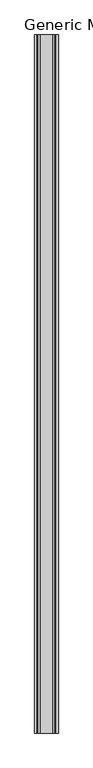
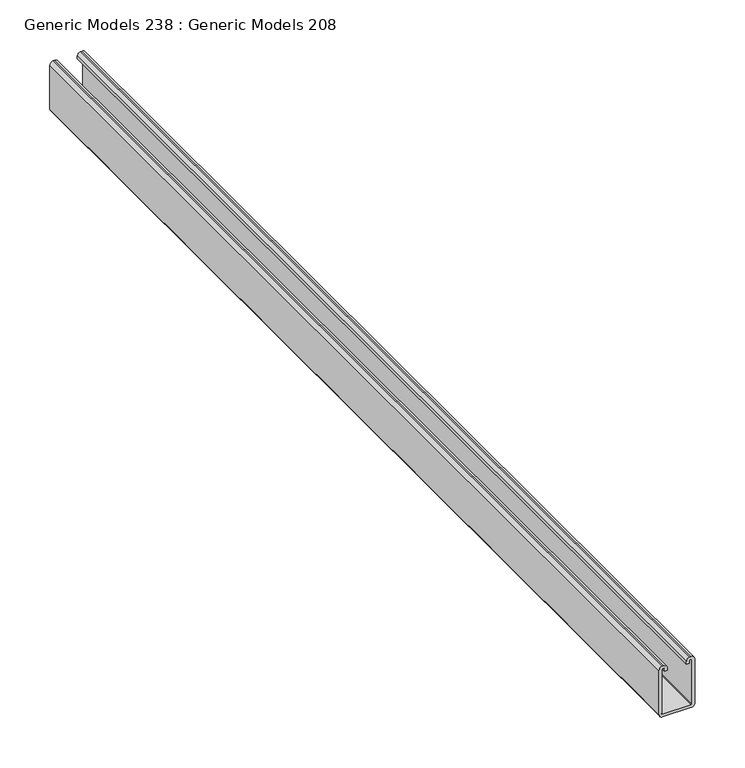
"""IFC4 building model written with IfcOpenShell, lengths in millimetres: proxy geometry, Generic Models 238 : Generic Models 208."""

from ifc_helpers import new_model, si_unit, point, frame, frame_2d, origin, place, context, project, spatial, polyline, circle_curve, trimmed, segment, composite_curve, outline, extrude, source, transform, mapped, element, save


def generic_models_238_generic_models_208_010beb91(model_context):
    return source(origin(), model_context, "Body", "SweptSolid", [
        extrude(outline(composite_curve([segment(polyline([(1885.7283045, 53737.481697), (1882.5378412, 53737.481697), (1882.5378412, 53740.656697), (1885.7283045, 53740.656697)]), True, "CONTINUOUS"), segment(trimmed(circle_curve(frame_2d((1885.7283045, 53741.4349838)), 0.7782868), [point((1885.7283045, 53740.656697))], [point((1886.5065912, 53741.4349838))], True, "CARTESIAN"), True, "CONTINUOUS"), segment(polyline([(1886.5065912, 53741.4349838), (1886.5065912, 53742.9812383)]), True, "CONTINUOUS"), segment(trimmed(circle_curve(frame_2d((1885.6561325, 53742.9812383)), 0.8504588), [point((1886.5065912, 53742.9812383))], [point((1885.6561325, 53743.831697))], True, "CARTESIAN"), True, "CONTINUOUS"), segment(polyline([(1885.6561325, 53743.831697), (1831.7929359, 53743.831697)]), True, "CONTINUOUS"), segment(trimmed(circle_curve(frame_2d((1831.7929359, 53742.9828524)), 0.8488446), [point((1831.7929359, 53743.831697))], [point((1830.9440912, 53742.9828524))], True, "CARTESIAN"), True, "CONTINUOUS"), segment(polyline([(1830.9440912, 53742.9828524), (1830.9440912, 53709.7160199)]), True, "CONTINUOUS"), segment(trimmed(circle_curve(frame_2d((1831.7534142, 53709.7160199)), 0.8093229), [point((1830.9440912, 53709.7160199))], [point((1831.7534142, 53708.906697))], True, "CARTESIAN"), True, "CONTINUOUS"), segment(polyline([(1831.7534142, 53708.906697), (1885.6696823, 53708.906697)]), True, "CONTINUOUS"), segment(trimmed(circle_curve(frame_2d((1885.6696823, 53709.7436059)), 0.8369089), [point((1885.6696823, 53708.906697))], [point((1886.5065912, 53709.7436059))], True, "CARTESIAN"), True, "CONTINUOUS"), segment(polyline([(1886.5065912, 53709.7436059), (1886.5065912, 53711.2123941)]), True, "CONTINUOUS"), segment(trimmed(circle_curve(frame_2d((1885.6372883, 53711.2123941)), 0.8693029), [point((1886.5065912, 53711.2123941))], [point((1885.6372883, 53712.081697))], True, "CARTESIAN"), True, "CONTINUOUS"), segment(polyline([(1885.6372883, 53712.081697), (1882.5378412, 53712.081697), (1882.5378412, 53715.256697), (1885.6372883, 53715.256697)]), True, "CONTINUOUS"), segment(trimmed(circle_curve(frame_2d((1885.6372883, 53711.2123941)), 4.0443029), [point((1885.6372883, 53715.256697))], [point((1889.6815912, 53711.2123941))], False, "CARTESIAN"), True, "CONTINUOUS"), segment(polyline([(1889.6815912, 53711.2123941), (1889.6815912, 53709.7436059)]), True, "CONTINUOUS"), segment(trimmed(circle_curve(frame_2d((1885.6696823, 53709.7436059)), 4.0119089), [point((1889.6815912, 53709.7436059))], [point((1885.6696823, 53705.731697))], False, "CARTESIAN"), True, "CONTINUOUS"), segment(polyline([(1885.6696823, 53705.731697), (1831.7534142, 53705.731697)]), True, "CONTINUOUS"), segment(trimmed(circle_curve(frame_2d((1831.7534142, 53709.7160199)), 3.9843229), [point((1831.7534142, 53705.731697))], [point((1827.7690912, 53709.7160199))], False, "CARTESIAN"), True, "CONTINUOUS"), segment(polyline([(1827.7690912, 53709.7160199), (1827.7690912, 53742.9828524)]), True, "CONTINUOUS"), segment(trimmed(circle_curve(frame_2d((1831.7929359, 53742.9828524)), 4.0238446), [point((1827.7690912, 53742.9828524))], [point((1831.7929359, 53747.006697))], False, "CARTESIAN"), True, "CONTINUOUS"), segment(polyline([(1831.7929359, 53747.006697), (1885.6561325, 53747.006697)]), True, "CONTINUOUS"), segment(trimmed(circle_curve(frame_2d((1885.6561325, 53742.9812383)), 4.0254588), [point((1885.6561325, 53747.006697))], [point((1889.6815912, 53742.9812383))], False, "CARTESIAN"), True, "CONTINUOUS"), segment(polyline([(1889.6815912, 53742.9812383), (1889.6815912, 53741.4349838)]), True, "CONTINUOUS"), segment(trimmed(circle_curve(frame_2d((1885.7283045, 53741.4349838)), 3.9532868), [point((1889.6815912, 53741.4349838))], [point((1885.7283045, 53737.481697))], False, "CARTESIAN"), True, "CONTINUOUS")], self_intersect=False)), frame((0.0, -228.7033818, 0.0), z_axis=(0.0, 1.0, 0.0), x_axis=(0.0, 0.0, 1.0)), (0.0, 0.0, 1.0), 1219.2),
    ])


if __name__ == "__main__":
    model = new_model("IFC4")
    model_context = context("Model", 3, world=origin())
    ifc_project = project(units=[si_unit("LENGTHUNIT", "METRE", prefix="MILLI")], contexts=[model_context])
    site = spatial("IfcSite", under=ifc_project)
    building = spatial("IfcBuilding", under=site)
    placement = place(None, origin())
    generic_models_238_generic_models_208_shape = generic_models_238_generic_models_208_010beb91(model_context)
    element("IfcBuildingElementProxy", 1, Name="Generic Models 238 : Generic Models 208", ObjectType="Generic Models 238 : Generic Models 208", at=placement, inside=building, context=model_context, shape_type="MappedRepresentation", body=[
        mapped(generic_models_238_generic_models_208_shape, transform((0.0, 0.0, 0.0), x_axis=(1.0, 0.0, 0.0), y_axis=(0.0, 1.0, 0.0), z_axis=(0.0, 0.0, 1.0))),
    ])
    save(model, "model.ifc")

# Revit data of these elements
# Element 1 (IfcBuildingElementProxy, "Generic Models 238 : Generic Models 208")
#   Materials on its faces: "GALVANIZED UNISTRUT P5500, 1 5/8\" X 2 7/16\" OR ALUM. CHANNEL"
# Materials
#   "GALVANIZED UNISTRUT P5500, 1 5/8\" X 2 7/16\" OR ALUM. CHANNEL": class "Metal", colour RGB 244 244 244, transparency 0, Description = "Aluminum 6061", Cost = 0
